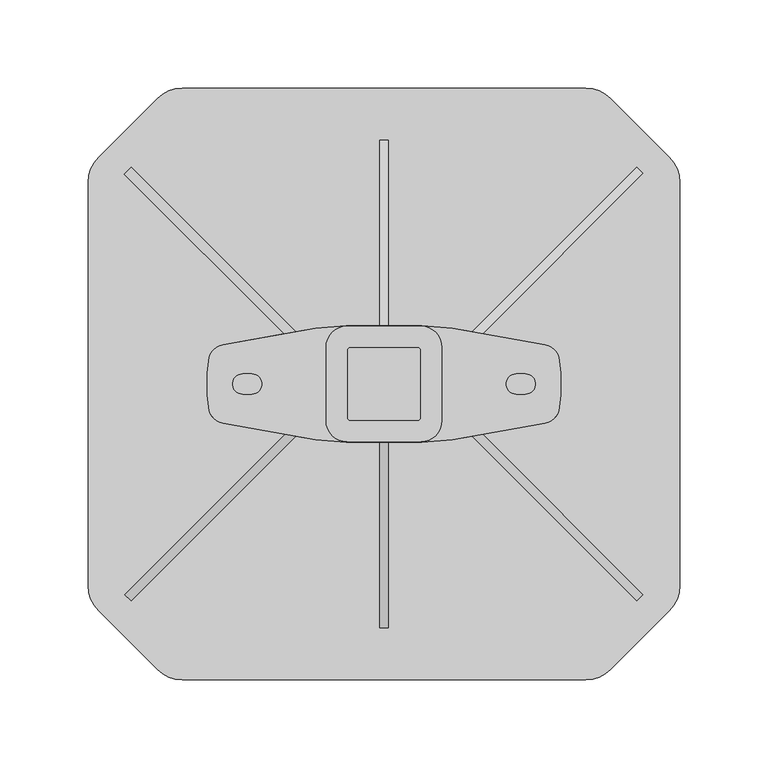
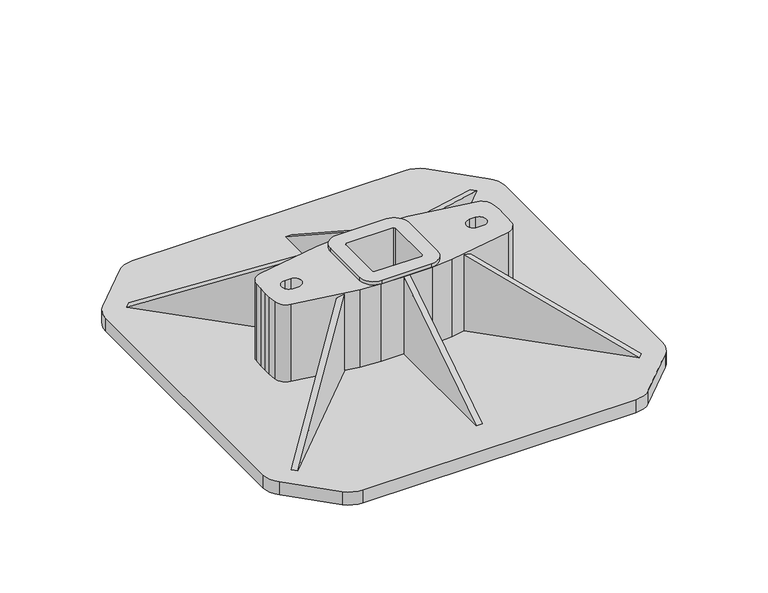
"""IFC4 building model written with IfcOpenShell, lengths in millimetres: proxy geometry, TN_Опора 335 B41-42 : Опора 335 B41/42."""

import ifcopenshell
import ifcopenshell.guid

model = None  # the IFC model being written
_history = None  # IfcOwnerHistory: only IFC2X3 demands one
_inside = {}  # id of a spatial element -> (the spatial element, [elements in it])
_under = {}  # id of a project, library or spatial element -> (it, [spatial elements below it])
_declared = {}  # id of a project -> (the project, [libraries it declares])
_typed = {}  # id of a type object -> (the type object, [elements of that type])
_made_of = {}  # id of a material, layer set ... -> (it, [elements and type objects made of it])


def new_model(schema):
    """Start an empty IFC model of exactly this schema.

    Asked for "IFC4X3", IfcOpenShell would pick the latest addendum, in which some entities
    have other attributes; the version numbers below select the first issue.
    IFC2X3 requires an IfcOwnerHistory on every rooted entity: one is made here for all.
    """
    global model, _history
    if schema == "IFC4X3":
        model = ifcopenshell.file(schema_version=(4, 3, 0, 0))
    else:
        model = ifcopenshell.file(schema=schema)
    _inside.clear()
    _under.clear()
    _declared.clear()
    _typed.clear()
    _made_of.clear()
    _history = None
    if model.schema == "IFC2X3":
        org = make("IfcOrganization", Name="unknown")
        user = make(
            "IfcPersonAndOrganization",
            ThePerson=make("IfcPerson", FamilyName="unknown"),
            TheOrganization=org,
        )
        app = make(
            "IfcApplication",
            ApplicationDeveloper=org,
            Version="unknown",
            ApplicationFullName="unknown",
            ApplicationIdentifier="unknown",
        )
        _history = make(
            "IfcOwnerHistory",
            OwningUser=user,
            OwningApplication=app,
            ChangeAction="ADDED",
            CreationDate=0,
        )
    return model


def make(cls, **values):
    """One entity of the class cls with the attributes given. An attribute that is None is left unset."""
    return model.create_entity(
        cls, **{name: value for name, value in values.items() if value is not None}
    )


def rooted(cls, **values):
    """An entity with a GlobalId (a new one), such as an element, a storey or a relation."""
    return make(cls, GlobalId=ifcopenshell.guid.new(), OwnerHistory=_history, **values)


def si_unit(unit_type, name, prefix=None):
    """IfcSIUnit, for example si_unit("LENGTHUNIT", "METRE", prefix="MILLI")."""
    return make("IfcSIUnit", UnitType=unit_type, Prefix=prefix, Name=name)


def assignment(units):
    """IfcUnitAssignment: the units of a project."""
    return None if units is None else make("IfcUnitAssignment", Units=units)


def point(xyz):
    """IfcCartesianPoint."""
    return None if xyz is None else make("IfcCartesianPoint", Coordinates=xyz)


def direction(xyz):
    """IfcDirection."""
    return None if xyz is None else make("IfcDirection", DirectionRatios=xyz)


def frame(location, z_axis=None, x_axis=None):
    """IfcAxis2Placement3D, a coordinate frame: its origin and axes. An axis left out is left unset."""
    return make(
        "IfcAxis2Placement3D",
        Location=point(location),
        Axis=direction(z_axis),
        RefDirection=direction(x_axis),
    )


def origin():
    """The frame at (0, 0, 0) with its axes left unset."""
    return frame((0.0, 0.0, 0.0))


def place(relative_to, where):
    """IfcLocalPlacement: puts the frame where relative to a parent placement (None: the world)."""
    return make(
        "IfcLocalPlacement", PlacementRelTo=relative_to, RelativePlacement=where
    )


def context(
    kind, dimensions, precision=None, world=None, true_north=None, identifier=None
):
    """IfcGeometricRepresentationContext, for example the 3D "Model" context."""
    return make(
        "IfcGeometricRepresentationContext",
        ContextIdentifier=identifier,
        ContextType=kind,
        CoordinateSpaceDimension=dimensions,
        Precision=precision,
        WorldCoordinateSystem=world,
        TrueNorth=true_north,
    )


def project(units=None, contexts=None):
    """IfcProject with its units and contexts."""
    return rooted(
        "IfcProject",
        Name="project",
        RepresentationContexts=contexts,
        UnitsInContext=assignment(units),
    )


def spatial(cls, under=None, at=None, **own):
    """A site, building, storey or space (cls), placed at a placement, below another one or the project."""
    s = rooted(cls, ObjectPlacement=at, **own)
    if under is not None:
        _under.setdefault(under.id(), (under, []))[1].append(s)
    return s


def polyline(points):
    """IfcPolyline through the points."""
    return make("IfcPolyline", Points=[point(p) for p in points])


def circle_curve(where, radius):
    """IfcCircle in the frame where."""
    return make("IfcCircle", Position=where, Radius=radius)


def shape(context_of_items, identifier, shape_type, items):
    """IfcShapeRepresentation: the items that make up one representation, for example the "Body"."""
    return make(
        "IfcShapeRepresentation",
        ContextOfItems=context_of_items,
        RepresentationIdentifier=identifier,
        RepresentationType=shape_type,
        Items=items,
    )


def source(mapping_origin, context_of_items, identifier, shape_type, items):
    """IfcRepresentationMap: a shape defined once, which mapped items show again and again."""
    return make(
        "IfcRepresentationMap",
        MappingOrigin=mapping_origin,
        MappedRepresentation=shape(context_of_items, identifier, shape_type, items),
    )


def transform(
    local_origin,
    x_axis=None,
    y_axis=None,
    z_axis=None,
    scale=None,
    scale2=None,
    scale3=None,
    uniform=True,
):
    """IfcCartesianTransformationOperator3D, or its non-uniform kind. x_axis, y_axis, z_axis: its Axis1, 2, 3."""
    if uniform:
        return make(
            "IfcCartesianTransformationOperator3D",
            Axis1=direction(x_axis),
            Axis2=direction(y_axis),
            LocalOrigin=point(local_origin),
            Scale=scale,
            Axis3=direction(z_axis),
        )
    return make(
        "IfcCartesianTransformationOperator3DnonUniform",
        Axis1=direction(x_axis),
        Axis2=direction(y_axis),
        LocalOrigin=point(local_origin),
        Scale=scale,
        Axis3=direction(z_axis),
        Scale2=scale2,
        Scale3=scale3,
    )


def mapped(mapping_source, mapping_target):
    """IfcMappedItem: shows the shape of a source again, moved by a transform."""
    return make(
        "IfcMappedItem", MappingSource=mapping_source, MappingTarget=mapping_target
    )


def made_of(thing, what):
    """Note that an element or type object is made of a material, layer set ...; save() writes the relation."""
    if what is not None:
        _made_of.setdefault(what.id(), (what, []))[1].append(thing)
    return thing


def element(
    cls,
    number,
    at=None,
    inside=None,
    cuts=None,
    type_object=None,
    material=None,
    context=None,
    identifier="Body",
    shape_type=None,
    held_by="IfcProductDefinitionShape",
    body=None,
    shapes=None,
    **own,
):
    """One element of the class cls, such as IfcWall. Its Tag is "e" and its number.

    at: its placement. inside: the storey or other place that contains it. cuts: it is an
    opening in that element (IfcRelVoidsElement). A single representation is given by context,
    identifier, shape_type and body (its items); several are given by shapes. held_by: the class
    of the entity that holds the representations. save() writes the other relations.
    """
    e = rooted(cls, Tag="e%d" % number, ObjectPlacement=at, **own)
    if body is not None:
        shapes = [shape(context, identifier, shape_type, body)]
    if shapes is not None:
        e.Representation = make(held_by, Representations=shapes)
    if inside is not None:
        _inside.setdefault(inside.id(), (inside, []))[1].append(e)
    if cuts is not None:
        rooted(
            "IfcRelVoidsElement", RelatingBuildingElement=cuts, RelatedOpeningElement=e
        )
    if type_object is not None:
        _typed.setdefault(type_object.id(), (type_object, []))[1].append(e)
    return made_of(e, material)


def aggregate(whole, parts):
    """IfcRelAggregates: a whole, such as a stair, and the parts it consists of."""
    return rooted("IfcRelAggregates", RelatingObject=whole, RelatedObjects=parts)


def save(model, path):
    """Write the relations noted so far, then the file.

    IfcRelAggregates (storeys below a building ...), IfcRelContainedInSpatialStructure (elements
    in a storey), IfcRelDefinesByType, IfcRelAssociatesMaterial and IfcRelDeclares: one each for
    every whole, place, type object, material and project.
    """
    for whole, parts in _under.values():
        aggregate(whole, parts)
    for where, things in _inside.values():
        rooted(
            "IfcRelContainedInSpatialStructure",
            RelatedElements=things,
            RelatingStructure=where,
        )
    for kind, things in _typed.values():
        rooted("IfcRelDefinesByType", RelatedObjects=things, RelatingType=kind)
    for what, things in _made_of.values():
        rooted("IfcRelAssociatesMaterial", RelatedObjects=things, RelatingMaterial=what)
    for by, libraries in _declared.values():
        rooted("IfcRelDeclares", RelatingContext=by, RelatedDefinitions=libraries)
    model.write(path)


def plane_surface(at):
    """IfcPlane: the flat surface through the origin of the frame at, square to its z axis."""
    return make("IfcPlane", Position=at)


def cylinder_surface(at, radius):
    """IfcCylindricalSurface: all points at the distance radius from the z axis of the frame at."""
    return make("IfcCylindricalSurface", Position=at, Radius=radius)


def revolved_surface(curve, axis_point, axis_direction):
    """IfcSurfaceOfRevolution: the curve turned about the line through axis_point along axis_direction."""
    return make(
        "IfcSurfaceOfRevolution",
        SweptCurve=make("IfcArbitraryOpenProfileDef", ProfileType="CURVE", Curve=curve),
        AxisPosition=make("IfcAxis1Placement", Location=point(axis_point), Axis=direction(axis_direction)),
    )


def advanced_brep(points, edges, surfaces, faces):
    """IfcAdvancedBrep: a solid bounded by faces that lie on surfaces and meet in shared edges.

    An edge is (start, end): straight between two places in points (the first is 0);
    or (start, end, curve); or (start, end, curve, False) where it runs against its curve.
    A face is (place in surfaces, loops), or (place, loops, False) where it looks against
    its surface's normal. A loop lists edges by number (the first is 1), with a minus sign
    where the edge is run from its end to its start. The first loop is the outer one.
    """
    corners = [point(p) for p in points]
    vertices = [make("IfcVertexPoint", VertexGeometry=c) for c in corners]
    made = []
    for start, end, *more in edges:
        made.append(
            make(
                "IfcEdgeCurve",
                EdgeStart=vertices[start],
                EdgeEnd=vertices[end],
                EdgeGeometry=more[0] if more else make("IfcPolyline", Points=[corners[start], corners[end]]),
                SameSense=more[1] if len(more) > 1 else True,
            )
        )
    hull = []
    for where, loops, *sense in faces:
        bounds = []
        for j, loop in enumerate(loops):
            ring = [make("IfcOrientedEdge", EdgeElement=made[abs(k) - 1], Orientation=k > 0) for k in loop]
            bounds.append(
                make(
                    "IfcFaceOuterBound" if j == 0 else "IfcFaceBound",
                    Bound=make("IfcEdgeLoop", EdgeList=ring),
                    Orientation=True,
                )
            )
        hull.append(make("IfcAdvancedFace", Bounds=bounds, FaceSurface=surfaces[where], SameSense=sense[0] if sense else True))
    return make("IfcAdvancedBrep", Outer=make("IfcClosedShell", CfsFaces=hull))


def generic_models_af6bc42f(model_context):
    return source(origin(), model_context, "Body", "AdvancedBrep", [
        advanced_brep(
        [(-23.35, -19.35, 11.5), (-23.35, 19.35, 11.5), (-19.35, 23.35, 11.5), (19.35, 23.35, 11.5), (23.35, 19.35, 11.5), (23.35, -19.35, 11.5), (19.35, -23.35, 11.5), (-19.35, -23.35, 11.5), (-19.5893398, 20.65, 11.5), (-20.65, 19.5893398, 11.5), (-20.65, -19.5893398, 11.5), (-19.5893398, -20.65, 11.5), (19.5893398, -20.65, 11.5), (20.65, -19.5893398, 11.5), (20.65, 19.5893398, 11.5), (19.5893398, 20.65, 11.5), (-19.35, -23.35, 80.0), (-23.35, -19.35, 80.0), (19.35, -23.35, 80.0), (23.35, -19.35, 80.0), (23.35, 19.35, 80.0), (19.35, 23.35, 80.0), (-19.35, 23.35, 80.0), (-23.35, 19.35, 80.0), (19.5893398, 20.65, 83.0), (-19.5893398, 20.65, 83.0), (20.65, 19.5893398, 83.0), (20.65, -19.5893398, 83.0), (19.5893398, -20.65, 83.0), (-19.5893398, -20.65, 83.0), (-20.65, -19.5893398, 83.0), (-20.65, 19.5893398, 83.0), (-32.8, 20.8, 83.0), (-32.8, -20.8, 83.0), (-20.8, -32.8, 83.0), (20.8, -32.8, 83.0), (32.8, -20.8, 83.0), (32.8, 20.8, 83.0), (20.8, 32.8, 83.0), (-20.8, 32.8, 83.0), (-32.8, 20.8, 80.0), (-20.8, 32.8, 80.0), (20.8, 32.8, 80.0), (32.8, 20.8, 80.0), (32.8, -20.8, 80.0), (20.8, -32.8, 80.0), (-20.8, -32.8, 80.0), (-32.8, -20.8, 80.0)],
        [
            (0, 1),
            (1, 2, circle_curve(frame((-19.35, 19.35, 11.5), z_axis=(0.0, 0.0, -1.0), x_axis=(1.0, 0.0, 0.0)), 4.0)),
            (2, 3),
            (3, 4, circle_curve(frame((19.35, 19.35, 11.5), z_axis=(0.0, 0.0, -1.0), x_axis=(1.0, 0.0, 0.0)), 4.0)),
            (4, 5),
            (5, 6, circle_curve(frame((19.35, -19.35, 11.5), z_axis=(0.0, 0.0, -1.0), x_axis=(1.0, 0.0, 0.0)), 4.0)),
            (6, 7),
            (7, 0, circle_curve(frame((-19.35, -19.35, 11.5), z_axis=(0.0, 0.0, -1.0), x_axis=(1.0, 0.0, 0.0)), 4.0)),
            (8, 9),
            (9, 10),
            (10, 11),
            (11, 12),
            (12, 13),
            (13, 14),
            (14, 15),
            (15, 8),
            (7, 16),
            (16, 17, circle_curve(frame((-19.35, -19.35, 80.0), z_axis=(0.0, 0.0, -1.0), x_axis=(1.0, 0.0, 0.0)), 4.0)),
            (17, 0),
            (6, 18),
            (18, 16),
            (5, 19),
            (19, 18, circle_curve(frame((19.35, -19.35, 80.0), z_axis=(0.0, 0.0, -1.0), x_axis=(1.0, 0.0, 0.0)), 4.0)),
            (4, 20),
            (20, 19),
            (3, 21),
            (21, 20, circle_curve(frame((19.35, 19.35, 80.0), z_axis=(0.0, 0.0, -1.0), x_axis=(1.0, 0.0, 0.0)), 4.0)),
            (2, 22),
            (22, 21),
            (1, 23),
            (23, 22, circle_curve(frame((-19.35, 19.35, 80.0), z_axis=(0.0, 0.0, -1.0), x_axis=(1.0, 0.0, 0.0)), 4.0)),
            (17, 23),
            (15, 24),
            (24, 25),
            (25, 8),
            (14, 26),
            (26, 24),
            (13, 27),
            (27, 26),
            (12, 28),
            (28, 27),
            (11, 29),
            (29, 28),
            (10, 30),
            (30, 29),
            (9, 31),
            (31, 30),
            (25, 31),
            (32, 33),
            (33, 34, circle_curve(frame((-20.8, -20.8, 83.0), z_axis=(0.0, 0.0, 1.0), x_axis=(1.0, 0.0, 0.0)), 12.0)),
            (34, 35),
            (35, 36, circle_curve(frame((20.8, -20.8, 83.0), z_axis=(0.0, 0.0, 1.0), x_axis=(1.0, 0.0, 0.0)), 12.0)),
            (36, 37),
            (37, 38, circle_curve(frame((20.8, 20.8, 83.0), z_axis=(0.0, 0.0, 1.0), x_axis=(1.0, 0.0, 0.0)), 12.0)),
            (38, 39),
            (39, 32, circle_curve(frame((-20.8, 20.8, 83.0), z_axis=(0.0, 0.0, 1.0), x_axis=(1.0, 0.0, 0.0)), 12.0)),
            (40, 41, circle_curve(frame((-20.8, 20.8, 80.0), z_axis=(0.0, 0.0, -1.0), x_axis=(1.0, 0.0, 0.0)), 12.0)),
            (41, 42),
            (42, 43, circle_curve(frame((20.8, 20.8, 80.0), z_axis=(0.0, 0.0, -1.0), x_axis=(1.0, 0.0, 0.0)), 12.0)),
            (43, 44),
            (44, 45, circle_curve(frame((20.8, -20.8, 80.0), z_axis=(0.0, 0.0, -1.0), x_axis=(1.0, 0.0, 0.0)), 12.0)),
            (45, 46),
            (46, 47, circle_curve(frame((-20.8, -20.8, 80.0), z_axis=(0.0, 0.0, -1.0), x_axis=(1.0, 0.0, 0.0)), 12.0)),
            (47, 40),
            (32, 40),
            (47, 33),
            (46, 34),
            (45, 35),
            (44, 36),
            (43, 37),
            (42, 38),
            (41, 39),
        ],
        [
            plane_surface(frame((-15.35, -19.35, 11.5), z_axis=(0.0, 0.0, -1.0), x_axis=(0.0, -1.0, 0.0))),
            cylinder_surface(frame((-19.35, -19.35, 11.5), z_axis=(0.0, 0.0, 1.0), x_axis=(1.0, 0.0, 0.0)), 4.0),
            plane_surface(frame((-19.35, -23.35, 80.0), z_axis=(0.0, -1.0, 0.0), x_axis=(0.0, 0.0, -1.0))),
            cylinder_surface(frame((19.35, -19.35, 11.5), z_axis=(0.0, 0.0, 1.0), x_axis=(1.0, 0.0, 0.0)), 4.0),
            plane_surface(frame((23.35, -19.35, 80.0), z_axis=(1.0, 0.0, 0.0), x_axis=(0.0, 0.0, -1.0))),
            cylinder_surface(frame((19.35, 19.35, 11.5), z_axis=(0.0, 0.0, 1.0), x_axis=(1.0, 0.0, 0.0)), 4.0),
            plane_surface(frame((19.35, 23.35, 80.0), z_axis=(0.0, 1.0, 0.0), x_axis=(0.0, 0.0, -1.0))),
            cylinder_surface(frame((-19.35, 19.35, 11.5), z_axis=(0.0, 0.0, 1.0), x_axis=(1.0, 0.0, 0.0)), 4.0),
            plane_surface(frame((-23.35, 19.35, 80.0), z_axis=(-1.0, 0.0, 0.0), x_axis=(0.0, 0.0, -1.0))),
            plane_surface(frame((-19.5893398, 20.65, 80.0), z_axis=(0.0, -1.0, 0.0), x_axis=(0.0, 0.0, -1.0))),
            plane_surface(frame((19.5893398, 20.65, 80.0), z_axis=(-0.7071067811865461, -0.707106781186549, 0.0), x_axis=(0.0, 0.0, -1.0))),
            plane_surface(frame((20.65, 19.5893398, 80.0), z_axis=(-1.0, 0.0, 0.0), x_axis=(0.0, 0.0, -1.0))),
            plane_surface(frame((20.65, -19.5893398, 80.0), z_axis=(-0.7071067811865461, 0.7071067811865489, 0.0), x_axis=(0.0, 0.0, -1.0))),
            plane_surface(frame((19.5893398, -20.65, 80.0), z_axis=(0.0, 1.0, 0.0), x_axis=(0.0, 0.0, -1.0))),
            plane_surface(frame((-19.5893398, -20.65, 80.0), z_axis=(0.707106781186549, 0.7071067811865461, 0.0), x_axis=(0.0, 0.0, -1.0))),
            plane_surface(frame((-20.65, -19.5893398, 80.0), z_axis=(1.0, 0.0, 0.0), x_axis=(0.0, 0.0, -1.0))),
            plane_surface(frame((-20.65, 19.5893398, 80.0), z_axis=(0.7071067811865476, -0.7071067811865476, 0.0), x_axis=(0.0, 0.0, -1.0))),
            plane_surface(frame((-20.65, 19.5893398, 83.0), z_axis=(0.0, 0.0, 1.0000000000000002), x_axis=(0.7071067811865462, 0.707106781186549, 0.0))),
            plane_surface(frame((-20.65, 19.5893398, 80.0), z_axis=(0.0, 0.0, -1.0000000000000002), x_axis=(-0.7071067811865462, -0.707106781186549, 0.0))),
            plane_surface(frame((-32.8, 20.8, 83.0), z_axis=(-1.0, 0.0, 0.0), x_axis=(0.0, 0.0, -1.0))),
            cylinder_surface(frame((-20.8, -20.8, 15.5), z_axis=(0.0, 0.0, 1.0), x_axis=(1.0, 0.0, 0.0)), 12.0),
            plane_surface(frame((-20.8, -32.8, 83.0), z_axis=(0.0, -1.0, 0.0), x_axis=(0.0, 0.0, -1.0))),
            cylinder_surface(frame((20.8, -20.8, 15.5), z_axis=(0.0, 0.0, 1.0), x_axis=(1.0, 0.0, 0.0)), 12.0),
            plane_surface(frame((32.8, -20.8, 83.0), z_axis=(1.0, 0.0, 0.0), x_axis=(0.0, 0.0, -1.0))),
            cylinder_surface(frame((20.8, 20.8, 15.5), z_axis=(0.0, 0.0, 1.0), x_axis=(1.0, 0.0, 0.0)), 12.0),
            plane_surface(frame((20.8, 32.8, 83.0), z_axis=(0.0, 1.0, 0.0), x_axis=(0.0, 0.0, -1.0))),
            cylinder_surface(frame((-20.8, 20.8, 15.5), z_axis=(0.0, 0.0, 1.0), x_axis=(1.0, 0.0, 0.0)), 12.0),
        ],
        [
            (0, [[1, 2, 3, 4, 5, 6, 7, 8], [9, 10, 11, 12, 13, 14, 15, 16]]),
            (1, [[-8, 17, 18, 19]]),
            (2, [[-7, 20, 21, -17]]),
            (3, [[-6, 22, 23, -20]]),
            (4, [[-5, 24, 25, -22]]),
            (5, [[-4, 26, 27, -24]]),
            (6, [[-3, 28, 29, -26]]),
            (7, [[-2, 30, 31, -28]]),
            (8, [[-1, -19, 32, -30]]),
            (9, [[-16, 33, 34, 35]]),
            (10, [[-33, -15, 36, 37]]),
            (11, [[-36, -14, 38, 39]]),
            (12, [[-38, -13, 40, 41]]),
            (13, [[-40, -12, 42, 43]]),
            (14, [[-42, -11, 44, 45]]),
            (15, [[-44, -10, 46, 47]]),
            (16, [[-46, -9, -35, 48]]),
            (17, [[49, 50, 51, 52, 53, 54, 55, 56], [-48, -34, -37, -39, -41, -43, -45, -47]]),
            (18, [[57, 58, 59, 60, 61, 62, 63, 64], [-18, -21, -23, -25, -27, -29, -31, -32]]),
            (19, [[-49, 65, -64, 66]]),
            (20, [[-50, -66, -63, 67]]),
            (21, [[-51, -67, -62, 68]]),
            (22, [[-52, -68, -61, 69]]),
            (23, [[-53, -69, -60, 70]]),
            (24, [[-54, -70, -59, 71]]),
            (25, [[-55, -71, -58, 72]]),
            (26, [[-56, -72, -57, -65]]),
        ],
    ),
        advanced_brep(
        [(-143.1614178, 122.7969517, 11.5), (-49.8622207, 29.4977546, 79.0270484), (-49.8622207, 29.4977546, 11.5), (-56.4807324, 28.3307324, 77.0542393), (-147.0541847, 118.9041847, 11.5), (-56.4807324, 28.3307324, 11.5), (21.2511336, -33.0, 80.0), (38.6159514, -31.4807753, 80.0), (91.1408813, -22.219213, 80.0), (99.3663465, -13.2426929, 80.0), (100.0, -6.0, 80.0), (100.0, 0.0, 80.0), (100.0, 6.0, 80.0), (99.3663465, 13.2426929, 80.0), (91.1408813, 22.219213, 80.0), (38.6159514, 31.4807753, 80.0), (21.2511336, 33.0, 80.0), (2.5, 33.0, 80.0), (0.0, 33.0, 80.0), (-2.5, 33.0, 80.0), (-21.2511336, 33.0, 80.0), (-38.6159514, 31.4807753, 80.0), (-91.1408813, 22.219213, 80.0), (-99.3663465, 13.2426929, 80.0), (-100.0, 6.0, 80.0), (-100.0, 0.0, 80.0), (-100.0, -6.0, 80.0), (-99.3663465, -13.2426929, 80.0), (-91.1408813, -22.219213, 80.0), (-38.6159514, -31.4807753, 80.0), (-21.2511336, -33.0, 80.0), (-2.5, -33.0, 80.0), (0.0, -33.0, 80.0), (2.5, -33.0, 80.0), (-80.0, -5.75, 80.0), (-80.0, 5.75, 80.0), (-75.0, 5.75, 80.0), (-75.0, -5.75, 80.0), (80.0, -5.75, 80.0), (75.0, -5.75, 80.0), (75.0, 5.75, 80.0), (80.0, 5.75, 80.0), (-4.25, 25.0, 80.0), (-4.25, 23.9, 80.0), (4.25, 23.9, 80.0), (4.25, 25.0, 80.0), (25.0, 25.0, 80.0), (25.0, 4.25, 80.0), (23.9, 4.25, 80.0), (23.9, -4.25, 80.0), (25.0, -4.25, 80.0), (25.0, -25.0, 80.0), (4.25, -25.0, 80.0), (4.25, -23.9, 80.0), (-4.25, -23.9, 80.0), (-4.25, -25.0, 80.0), (-25.0, -25.0, 80.0), (-25.0, -4.25, 80.0), (-23.9, -4.25, 80.0), (-23.9, 4.25, 80.0), (-25.0, 4.25, 80.0), (-25.0, 25.0, 80.0), (-80.0, -5.75, 11.5), (-80.0, 5.75, 11.5), (-75.0, 5.75, 11.5), (-75.0, -5.75, 11.5), (80.0, -5.75, 11.5), (75.0, -5.75, 11.5), (75.0, 5.75, 11.5), (80.0, 5.75, 11.5), (-21.2511336, -33.0, 11.5), (-2.5, -33.0, 11.5), (21.2511336, -33.0, 11.5), (2.5, -33.0, 11.5), (38.6159514, -31.4807753, 11.5), (49.8622207, -29.4977546, 11.5), (49.8622207, -29.4977546, 79.0270484), (55.8733621, -28.4378282, 77.2352809), (55.8733621, -28.4378282, 11.5), (91.1408813, -22.219213, 11.5), (99.3663465, -13.2426929, 11.5), (100.0, -6.0, 11.5), (100.0, 0.0, 11.5), (100.0, 6.0, 11.5), (99.3663465, 13.2426929, 11.5), (91.1408813, 22.219213, 11.5), (55.8733621, 28.4378282, 11.5), (55.8733621, 28.4378282, 77.2352809), (49.8622207, 29.4977546, 79.0270484), (49.8622207, 29.4977546, 11.5), (38.6159514, 31.4807753, 11.5), (21.2511336, 33.0, 11.5), (2.5, 33.0, 11.5), (-21.2511336, 33.0, 11.5), (-2.5, 33.0, 11.5), (-38.6159514, 31.4807753, 11.5), (-91.1408813, 22.219213, 11.5), (-99.3663465, 13.2426929, 11.5), (-100.0, 6.0, 11.5), (-100.0, 0.0, 11.5), (-100.0, -6.0, 11.5), (-99.3663465, -13.2426929, 11.5), (-91.1408813, -22.219213, 11.5), (-55.8733621, -28.4378282, 11.5), (-55.8733621, -28.4378282, 77.2352809), (-49.8622207, -29.4977546, 79.0270484), (-49.8622207, -29.4977546, 11.5), (-38.6159514, -31.4807753, 11.5), (-4.25, 25.0, 11.5), (-4.25, 23.9, 11.5), (4.25, 23.9, 11.5), (4.25, 25.0, 11.5), (25.0, 25.0, 11.5), (25.0, 4.25, 11.5), (23.9, 4.25, 11.5), (23.9, -4.25, 11.5), (25.0, -4.25, 11.5), (25.0, -25.0, 11.5), (4.25, -25.0, 11.5), (4.25, -23.9, 11.5), (-4.25, -23.9, 11.5), (-4.25, -25.0, 11.5), (-25.0, -25.0, 11.5), (-25.0, -4.25, 11.5), (-23.9, -4.25, 11.5), (-23.9, 4.25, 11.5), (-25.0, 4.25, 11.5), (-25.0, 25.0, 11.5), (2.5, 138.0, 11.5), (-2.5, 138.0, 11.5), (143.1614178, 122.7969517, 11.5), (146.6969517, 119.2614178, 11.5), (143.1614178, -122.7969517, 11.5), (146.6969517, -119.2614178, 11.5), (2.5, -138.0, 11.5), (-2.5, -138.0, 11.5), (-143.1614178, -122.7969517, 11.5), (-146.6969517, -119.2614178, 11.5), (114.2157288, 167.5, 11.5), (-114.2157288, 167.5, 11.5), (-128.3578644, 161.6421356, 11.5), (-161.6421356, 128.3578644, 11.5), (-167.5, 114.2157288, 11.5), (-167.5, -114.2157288, 11.5), (-161.6421356, -128.3578644, 11.5), (-128.3578644, -161.6421356, 11.5), (-114.2157288, -167.5, 11.5), (114.2157288, -167.5, 11.5), (128.3578644, -161.6421356, 11.5), (161.6421356, -128.3578644, 11.5), (167.5, -114.2157288, 11.5), (167.5, 114.2157288, 11.5), (161.6421356, 128.3578644, 11.5), (128.3578644, 161.6421356, 11.5), (114.2157288, 167.5, 0.0), (128.3578644, 161.6421356, 0.0), (161.6421356, 128.3578644, 0.0), (167.5, 114.2157288, 0.0), (167.5, -114.2157288, 0.0), (161.6421356, -128.3578644, 0.0), (128.3578644, -161.6421356, 0.0), (114.2157288, -167.5, 0.0), (-114.2157288, -167.5, 0.0), (-128.3578644, -161.6421356, 0.0), (-161.6421356, -128.3578644, 0.0), (-167.5, -114.2157288, 0.0), (-167.5, 114.2157288, 0.0), (-161.6421356, 128.3578644, 0.0), (-128.3578644, 161.6421356, 0.0), (-114.2157288, 167.5, 0.0)],
        [
            (0, 1),
            (1, 2),
            (2, 0),
            (3, 4),
            (4, 5),
            (5, 3),
            (0, 4),
            (3, 1),
            (6, 7, circle_curve(frame((21.2511336, 67.0, 80.0), z_axis=(0.0, 0.0, 1.0), x_axis=(1.0, 0.0, 0.0)), 100.0)),
            (7, 8),
            (8, 9, circle_curve(frame((89.4043995, -12.3711355, 80.0), z_axis=(0.0, 0.0, 1.0), x_axis=(1.0, 0.0, 0.0)), 10.0)),
            (9, 10),
            (10, 11),
            (11, 12),
            (12, 13),
            (13, 14, circle_curve(frame((89.4043995, 12.3711355, 80.0), z_axis=(0.0, 0.0, 1.0), x_axis=(1.0, 0.0, 0.0)), 10.0)),
            (14, 15),
            (15, 16, circle_curve(frame((21.2511336, -67.0, 80.0), z_axis=(0.0, 0.0, 1.0), x_axis=(1.0, 0.0, 0.0)), 100.0)),
            (16, 17),
            (17, 18),
            (18, 19),
            (19, 20),
            (20, 21, circle_curve(frame((-21.2511336, -67.0, 80.0), z_axis=(0.0, 0.0, 1.0), x_axis=(1.0, 0.0, 0.0)), 100.0)),
            (21, 22),
            (22, 23, circle_curve(frame((-89.4043995, 12.3711355, 80.0), z_axis=(0.0, 0.0, 1.0), x_axis=(1.0, 0.0, 0.0)), 10.0)),
            (23, 24),
            (24, 25),
            (25, 26),
            (26, 27),
            (27, 28, circle_curve(frame((-89.4043995, -12.3711355, 80.0), z_axis=(0.0, 0.0, 1.0), x_axis=(1.0, 0.0, 0.0)), 10.0)),
            (28, 29),
            (29, 30, circle_curve(frame((-21.2511336, 67.0, 80.0), z_axis=(0.0, 0.0, 1.0), x_axis=(1.0, 0.0, 0.0)), 100.0)),
            (30, 31),
            (31, 32),
            (32, 33),
            (33, 6),
            (34, 35, circle_curve(frame((-80.0, 0.0, 80.0), z_axis=(0.0, 0.0, -1.0), x_axis=(1.0, 0.0, 0.0)), 5.75)),
            (35, 36),
            (36, 37, circle_curve(frame((-75.0, 0.0, 80.0), z_axis=(0.0, 0.0, -1.0), x_axis=(1.0, 0.0, 0.0)), 5.75)),
            (37, 34),
            (38, 39),
            (39, 40, circle_curve(frame((75.0, 0.0, 80.0), z_axis=(0.0, 0.0, -1.0), x_axis=(1.0, 0.0, 0.0)), 5.75)),
            (40, 41),
            (41, 38, circle_curve(frame((80.0, 0.0, 80.0), z_axis=(0.0, 0.0, -1.0), x_axis=(1.0, 0.0, 0.0)), 5.75)),
            (42, 43),
            (43, 44),
            (44, 45),
            (45, 46),
            (46, 47),
            (47, 48),
            (48, 49),
            (49, 50),
            (50, 51),
            (51, 52),
            (52, 53),
            (53, 54),
            (54, 55),
            (55, 56),
            (56, 57),
            (57, 58),
            (58, 59),
            (59, 60),
            (60, 61),
            (61, 42),
            (34, 62),
            (62, 63, circle_curve(frame((-80.0, 0.0, 11.5), z_axis=(0.0, 0.0, -1.0), x_axis=(1.0, 0.0, 0.0)), 5.75)),
            (63, 35),
            (63, 64),
            (64, 36),
            (64, 65, circle_curve(frame((-75.0, 0.0, 11.5), z_axis=(0.0, 0.0, -1.0), x_axis=(1.0, 0.0, 0.0)), 5.75)),
            (65, 37),
            (65, 62),
            (38, 66),
            (66, 67),
            (67, 39),
            (67, 68, circle_curve(frame((75.0, 0.0, 11.5), z_axis=(0.0, 0.0, -1.0), x_axis=(1.0, 0.0, 0.0)), 5.75)),
            (68, 40),
            (68, 69),
            (69, 41),
            (69, 66, circle_curve(frame((80.0, 0.0, 11.5), z_axis=(0.0, 0.0, -1.0), x_axis=(1.0, 0.0, 0.0)), 5.75)),
            (30, 70),
            (70, 71),
            (71, 31),
            (72, 6),
            (33, 73),
            (73, 72),
            (72, 74, circle_curve(frame((21.2511336, 67.0, 11.5), z_axis=(0.0, 0.0, 1.0), x_axis=(1.0, 0.0, 0.0)), 100.0)),
            (74, 7),
            (74, 75),
            (75, 76),
            (76, 77),
            (77, 78),
            (78, 79),
            (79, 8),
            (79, 80, circle_curve(frame((89.4043995, -12.3711355, 11.5), z_axis=(0.0, 0.0, 1.0), x_axis=(1.0, 0.0, 0.0)), 10.0)),
            (80, 9),
            (80, 81),
            (81, 10),
            (81, 82),
            (82, 11),
            (82, 83),
            (83, 12),
            (83, 84),
            (84, 13),
            (84, 85, circle_curve(frame((89.4043995, 12.3711355, 11.5), z_axis=(0.0, 0.0, 1.0), x_axis=(1.0, 0.0, 0.0)), 10.0)),
            (85, 14),
            (85, 86),
            (86, 87),
            (87, 88),
            (88, 89),
            (89, 90),
            (90, 15),
            (90, 91, circle_curve(frame((21.2511336, -67.0, 11.5), z_axis=(0.0, 0.0, 1.0), x_axis=(1.0, 0.0, 0.0)), 100.0)),
            (91, 16),
            (91, 92),
            (92, 17),
            (93, 20),
            (19, 94),
            (94, 93),
            (93, 95, circle_curve(frame((-21.2511336, -67.0, 11.5), z_axis=(0.0, 0.0, 1.0), x_axis=(1.0, 0.0, 0.0)), 100.0)),
            (95, 21),
            (95, 2),
            (5, 96),
            (96, 22),
            (96, 97, circle_curve(frame((-89.4043995, 12.3711355, 11.5), z_axis=(0.0, 0.0, 1.0), x_axis=(1.0, 0.0, 0.0)), 10.0)),
            (97, 23),
            (97, 98),
            (98, 24),
            (98, 99),
            (99, 25),
            (99, 100),
            (100, 26),
            (100, 101),
            (101, 27),
            (101, 102, circle_curve(frame((-89.4043995, -12.3711355, 11.5), z_axis=(0.0, 0.0, 1.0), x_axis=(1.0, 0.0, 0.0)), 10.0)),
            (102, 28),
            (102, 103),
            (103, 104),
            (104, 105),
            (105, 106),
            (106, 107),
            (107, 29),
            (107, 70, circle_curve(frame((-21.2511336, 67.0, 11.5), z_axis=(0.0, 0.0, 1.0), x_axis=(1.0, 0.0, 0.0)), 100.0)),
            (42, 108),
            (108, 109),
            (109, 43),
            (109, 110),
            (110, 44),
            (110, 111),
            (111, 45),
            (111, 112),
            (112, 46),
            (112, 113),
            (113, 47),
            (113, 114),
            (114, 48),
            (114, 115),
            (115, 49),
            (115, 116),
            (116, 50),
            (116, 117),
            (117, 51),
            (117, 118),
            (118, 52),
            (118, 119),
            (119, 53),
            (119, 120),
            (120, 54),
            (120, 121),
            (121, 55),
            (121, 122),
            (122, 56),
            (122, 123),
            (123, 57),
            (123, 124),
            (124, 58),
            (124, 125),
            (125, 59),
            (125, 126),
            (126, 60),
            (126, 127),
            (127, 61),
            (127, 108),
            (128, 17),
            (92, 128),
            (19, 129),
            (129, 94),
            (128, 129),
            (88, 130),
            (130, 89),
            (131, 87),
            (86, 131),
            (131, 130),
            (132, 76),
            (75, 132),
            (77, 133),
            (133, 78),
            (132, 133),
            (33, 134),
            (134, 73),
            (135, 31),
            (71, 135),
            (135, 134),
            (105, 136),
            (136, 106),
            (137, 104),
            (103, 137),
            (137, 136),
            (138, 139),
            (139, 140, circle_curve(frame((-114.2157288, 147.5, 11.5), z_axis=(0.0, 0.0, 1.0), x_axis=(1.0, 0.0, 0.0)), 20.0)),
            (140, 141),
            (141, 142, circle_curve(frame((-147.5, 114.2157288, 11.5), z_axis=(0.0, 0.0, 1.0), x_axis=(1.0, 0.0, 0.0)), 20.0)),
            (142, 143),
            (143, 144, circle_curve(frame((-147.5, -114.2157288, 11.5), z_axis=(0.0, 0.0, 1.0), x_axis=(1.0, 0.0, 0.0)), 20.0)),
            (144, 145),
            (145, 146, circle_curve(frame((-114.2157288, -147.5, 11.5), z_axis=(0.0, 0.0, 1.0), x_axis=(1.0, 0.0, 0.0)), 20.0)),
            (146, 147),
            (147, 148, circle_curve(frame((114.2157288, -147.5, 11.5), z_axis=(0.0, 0.0, 1.0), x_axis=(1.0, 0.0, 0.0)), 20.0)),
            (148, 149),
            (149, 150, circle_curve(frame((147.5, -114.2157288, 11.5), z_axis=(0.0, 0.0, 1.0), x_axis=(1.0, 0.0, 0.0)), 20.0)),
            (150, 151),
            (151, 152, circle_curve(frame((147.5, 114.2157288, 11.5), z_axis=(0.0, 0.0, 1.0), x_axis=(1.0, 0.0, 0.0)), 20.0)),
            (152, 153),
            (153, 138, circle_curve(frame((114.2157288, 147.5, 11.5), z_axis=(0.0, 0.0, 1.0), x_axis=(1.0, 0.0, 0.0)), 20.0)),
            (154, 155, circle_curve(frame((114.2157288, 147.5, 0.0), z_axis=(0.0, 0.0, -1.0), x_axis=(1.0, 0.0, 0.0)), 20.0)),
            (155, 156),
            (156, 157, circle_curve(frame((147.5, 114.2157288, 0.0), z_axis=(0.0, 0.0, -1.0), x_axis=(1.0, 0.0, 0.0)), 20.0)),
            (157, 158),
            (158, 159, circle_curve(frame((147.5, -114.2157288, 0.0), z_axis=(0.0, 0.0, -1.0), x_axis=(1.0, 0.0, 0.0)), 20.0)),
            (159, 160),
            (160, 161, circle_curve(frame((114.2157288, -147.5, 0.0), z_axis=(0.0, 0.0, -1.0), x_axis=(1.0, 0.0, 0.0)), 20.0)),
            (161, 162),
            (162, 163, circle_curve(frame((-114.2157288, -147.5, 0.0), z_axis=(0.0, 0.0, -1.0), x_axis=(1.0, 0.0, 0.0)), 20.0)),
            (163, 164),
            (164, 165, circle_curve(frame((-147.5, -114.2157288, 0.0), z_axis=(0.0, 0.0, -1.0), x_axis=(1.0, 0.0, 0.0)), 20.0)),
            (165, 166),
            (166, 167, circle_curve(frame((-147.5, 114.2157288, 0.0), z_axis=(0.0, 0.0, -1.0), x_axis=(1.0, 0.0, 0.0)), 20.0)),
            (167, 168),
            (168, 169, circle_curve(frame((-114.2157288, 147.5, 0.0), z_axis=(0.0, 0.0, -1.0), x_axis=(1.0, 0.0, 0.0)), 20.0)),
            (169, 154),
            (138, 154),
            (169, 139),
            (140, 168),
            (167, 141),
            (142, 166),
            (165, 143),
            (144, 164),
            (163, 145),
            (146, 162),
            (161, 147),
            (148, 160),
            (159, 149),
            (150, 158),
            (157, 151),
            (152, 156),
            (155, 153),
        ],
        [
            plane_surface(frame((-143.1614178, 122.7969517, 11.5), z_axis=(0.7071067811865471, 0.707106781186548, 0.0), x_axis=(0.6294612213167056, -0.6294612213167048, 0.4555843958225127))),
            plane_surface(frame((-147.0541847, 118.9041847, 11.5), z_axis=(-0.7071067811865471, -0.707106781186548, 0.0), x_axis=(-0.6294612213167056, 0.6294612213167048, -0.4555843958225127))),
            plane_surface(frame((-143.1614178, 122.7969517, 11.5), z_axis=(-0.322146815688875, 0.322146815688875, 0.8901925961740168), x_axis=(-0.7071067811865476, -0.7071067811865476, 0.0))),
            plane_surface(frame((-74.25, 0.0, 80.0), z_axis=(0.0, 0.0, 1.0), x_axis=(0.0, -1.0, 0.0))),
            revolved_surface(polyline([(-74.25, 0.0, 11.5), (-74.25, 0.0, 80.0)]), (-80.0, 0.0, 11.5), (0.0, 0.0, -1.0)),
            plane_surface(frame((-80.0, 5.75, 80.0), z_axis=(0.0, -1.0, 0.0), x_axis=(0.0, 0.0, -1.0))),
            revolved_surface(polyline([(-69.25, 0.0, 11.5), (-69.25, 0.0, 80.0)]), (-75.0, 0.0, 11.5), (0.0, 0.0, -1.0)),
            plane_surface(frame((-75.0, -5.75, 80.0), z_axis=(0.0, 1.0, 0.0), x_axis=(0.0, 0.0, -1.0))),
            plane_surface(frame((80.0, -5.75, 80.0), z_axis=(0.0, 1.0, 0.0), x_axis=(0.0, 0.0, -1.0))),
            revolved_surface(polyline([(80.75, 0.0, 11.5), (80.75, 0.0, 80.0)]), (75.0, 0.0, 0.0), (0.0, 0.0, -1.0)),
            plane_surface(frame((75.0, 5.75, 80.0), z_axis=(0.0, -1.0, 0.0), x_axis=(0.0, 0.0, -1.0))),
            revolved_surface(polyline([(85.75, 0.0, 11.5), (85.75, 0.0, 80.0)]), (80.0, 0.0, 0.0), (0.0, 0.0, -1.0)),
            plane_surface(frame((-21.2511336, -33.0, 80.0), z_axis=(0.0, -1.0, 0.0), x_axis=(0.0, 0.0, -1.0))),
            plane_surface(frame((0.0, -33.0, 80.0), z_axis=(0.0, -1.0, 0.0), x_axis=(0.0, 0.0, -1.0))),
            cylinder_surface(frame((21.2511336, 67.0, 0.0), z_axis=(0.0, 0.0, 1.0), x_axis=(1.0, 0.0, 0.0)), 100.0),
            plane_surface(frame((38.6159514, -31.4807753, 80.0), z_axis=(0.17364817766693338, -0.9848077530122076, 0.0), x_axis=(0.0, 0.0, -1.0))),
            cylinder_surface(frame((89.4043995, -12.3711355, 0.0), z_axis=(0.0, 0.0, 1.0), x_axis=(1.0, 0.0, 0.0)), 10.0),
            plane_surface(frame((99.3663465, -13.2426929, 80.0), z_axis=(0.9961946980917454, -0.08715574274765994, 0.0), x_axis=(0.0, 0.0, -1.0))),
            plane_surface(frame((100.0, -6.0, 80.0), z_axis=(1.0, 0.0, 0.0), x_axis=(0.0, 0.0, -1.0))),
            plane_surface(frame((100.0, 0.0, 80.0), z_axis=(1.0, 0.0, 0.0), x_axis=(0.0, 0.0, -1.0))),
            plane_surface(frame((100.0, 6.0, 80.0), z_axis=(0.9961946980917457, 0.08715574274765747, 0.0), x_axis=(0.0, 0.0, -1.0))),
            cylinder_surface(frame((89.4043995, 12.3711355, 0.0), z_axis=(0.0, 0.0, 1.0), x_axis=(1.0, 0.0, 0.0)), 10.0),
            plane_surface(frame((91.1408813, 22.219213, 80.0), z_axis=(0.17364817766693313, 0.9848077530122076, 0.0), x_axis=(0.0, 0.0, -1.0))),
            cylinder_surface(frame((21.2511336, -67.0, 0.0), z_axis=(0.0, 0.0, 1.0), x_axis=(1.0, 0.0, 0.0)), 100.0),
            plane_surface(frame((21.2511336, 33.0, 80.0), z_axis=(0.0, 1.0, 0.0), x_axis=(0.0, 0.0, -1.0))),
            plane_surface(frame((0.0, 33.0, 80.0), z_axis=(0.0, 1.0, 0.0), x_axis=(0.0, 0.0, -1.0))),
            cylinder_surface(frame((-21.2511336, -67.0, 0.0), z_axis=(0.0, 0.0, 1.0), x_axis=(1.0, 0.0, 0.0)), 100.0),
            plane_surface(frame((-38.6159514, 31.4807753, 80.0), z_axis=(-0.17364817766693333, 0.9848077530122076, 0.0), x_axis=(0.0, 0.0, -1.0))),
            cylinder_surface(frame((-89.4043995, 12.3711355, 0.0), z_axis=(0.0, 0.0, 1.0), x_axis=(1.0, 0.0, 0.0)), 10.0),
            plane_surface(frame((-99.3663465, 13.2426929, 80.0), z_axis=(-0.9961946980917454, 0.08715574274765955, 0.0), x_axis=(0.0, 0.0, -1.0))),
            plane_surface(frame((-100.0, 6.0, 80.0), z_axis=(-1.0, 0.0, 0.0), x_axis=(0.0, 0.0, -1.0))),
            plane_surface(frame((-100.0, 0.0, 80.0), z_axis=(-1.0, 0.0, 0.0), x_axis=(0.0, 0.0, -1.0))),
            plane_surface(frame((-100.0, -6.0, 80.0), z_axis=(-0.9961946980917455, -0.08715574274765889, 0.0), x_axis=(0.0, 0.0, -1.0))),
            cylinder_surface(frame((-89.4043995, -12.3711355, 0.0), z_axis=(0.0, 0.0, 1.0), x_axis=(1.0, 0.0, 0.0)), 10.0),
            plane_surface(frame((-91.1408813, -22.219213, 80.0), z_axis=(-0.17364817766693322, -0.9848077530122076, 0.0), x_axis=(0.0, 0.0, -1.0))),
            cylinder_surface(frame((-21.2511336, 67.0, 0.0), z_axis=(0.0, 0.0, 1.0), x_axis=(1.0, 0.0, 0.0)), 100.0),
            plane_surface(frame((-4.25, 25.0, 80.0), z_axis=(-1.0, 0.0, 0.0), x_axis=(0.0, 0.0, -1.0))),
            plane_surface(frame((-4.25, 23.9, 80.0), z_axis=(0.0, -1.0, 0.0), x_axis=(0.0, 0.0, -1.0))),
            plane_surface(frame((4.25, 23.9, 80.0), z_axis=(1.0, 0.0, 0.0), x_axis=(0.0, 0.0, -1.0))),
            plane_surface(frame((4.25, 25.0, 80.0), z_axis=(0.0, -1.0, 0.0), x_axis=(0.0, 0.0, -1.0))),
            plane_surface(frame((25.0, 25.0, 80.0), z_axis=(-1.0, 0.0, 0.0), x_axis=(0.0, 0.0, -1.0))),
            plane_surface(frame((25.0, 4.25, 80.0), z_axis=(0.0, 1.0, 0.0), x_axis=(0.0, 0.0, -1.0))),
            plane_surface(frame((23.9, 4.25, 80.0), z_axis=(-1.0, 0.0, 0.0), x_axis=(0.0, 0.0, -1.0))),
            plane_surface(frame((23.9, -4.25, 80.0), z_axis=(0.0, -1.0, 0.0), x_axis=(0.0, 0.0, -1.0))),
            plane_surface(frame((25.0, -4.25, 80.0), z_axis=(-1.0, 0.0, 0.0), x_axis=(0.0, 0.0, -1.0))),
            plane_surface(frame((25.0, -25.0, 80.0), z_axis=(0.0, 1.0, 0.0), x_axis=(0.0, 0.0, -1.0))),
            plane_surface(frame((4.25, -25.0, 80.0), z_axis=(1.0, 0.0, 0.0), x_axis=(0.0, 0.0, -1.0))),
            plane_surface(frame((4.25, -23.9, 80.0), z_axis=(0.0, 1.0, 0.0), x_axis=(0.0, 0.0, -1.0))),
            plane_surface(frame((-4.25, -23.9, 80.0), z_axis=(-1.0, 0.0, 0.0), x_axis=(0.0, 0.0, -1.0))),
            plane_surface(frame((-4.25, -25.0, 80.0), z_axis=(0.0, 1.0, 0.0), x_axis=(0.0, 0.0, -1.0))),
            plane_surface(frame((-25.0, -25.0, 80.0), z_axis=(1.0, 0.0, 0.0), x_axis=(0.0, 0.0, -1.0))),
            plane_surface(frame((-25.0, -4.25, 80.0), z_axis=(0.0, -1.0, 0.0), x_axis=(0.0, 0.0, -1.0))),
            plane_surface(frame((-23.9, -4.25, 80.0), z_axis=(1.0, 0.0, 0.0), x_axis=(0.0, 0.0, -1.0))),
            plane_surface(frame((-23.9, 4.25, 80.0), z_axis=(0.0, 1.0, 0.0), x_axis=(0.0, 0.0, -1.0))),
            plane_surface(frame((-25.0, 4.25, 80.0), z_axis=(1.0, 0.0, 0.0), x_axis=(0.0, 0.0, -1.0))),
            plane_surface(frame((-25.0, 25.0, 80.0), z_axis=(0.0, -1.0, 0.0), x_axis=(0.0, 0.0, -1.0))),
            plane_surface(frame((2.5, 138.0, 11.5), z_axis=(1.0, 0.0, 0.0), x_axis=(0.0, -0.8375312462789268, 0.5463894320962547))),
            plane_surface(frame((-2.5, 138.0, 11.5), z_axis=(-1.0, 0.0, 0.0), x_axis=(0.0, 0.8375312462789268, -0.5463894320962547))),
            plane_surface(frame((2.5, 138.0, 11.5), z_axis=(0.0, 0.5463894320962547, 0.8375312462789268), x_axis=(-1.0, 0.0, 0.0))),
            plane_surface(frame((65.3796718, 45.0152057, 11.5), z_axis=(-0.7071067811865471, 0.707106781186548, 0.0), x_axis=(-0.707106781186548, -0.7071067811865471, 0.0))),
            plane_surface(frame((68.9152057, 41.4796718, 11.5), z_axis=(0.7071067811865471, -0.707106781186548, 0.0), x_axis=(0.707106781186548, 0.7071067811865471, 0.0))),
            plane_surface(frame((48.5179356, 28.1534695, 80.0), z_axis=(0.3221468156888753, 0.32214681568887454, 0.8901925961740168), x_axis=(0.7071067811865467, -0.7071067811865483, 0.0))),
            plane_surface(frame((48.5179356, -28.1534695, 80.0), z_axis=(-0.707106781186547, -0.7071067811865481, 0.0), x_axis=(-0.6294612213167055, 0.6294612213167045, 0.4555843958225132))),
            plane_surface(frame((52.0534695, -24.6179356, 80.0), z_axis=(0.707106781186547, 0.7071067811865481, 0.0), x_axis=(0.6294612213167055, -0.6294612213167045, -0.4555843958225132))),
            plane_surface(frame((143.1614178, -122.7969517, 11.5), z_axis=(0.3221468156888754, -0.3221468156888754, 0.8901925961740167), x_axis=(0.7071067811865476, 0.7071067811865476, 0.0))),
            plane_surface(frame((2.5, -33.0, 11.5), z_axis=(1.0, 0.0, 0.0), x_axis=(0.0, 1.0, 0.0))),
            plane_surface(frame((-2.5, -33.0, 11.5), z_axis=(-1.0, 0.0, 0.0), x_axis=(0.0, -1.0, 0.0))),
            plane_surface(frame((2.5, -33.0, 80.0), z_axis=(0.0, -0.5463894320962547, 0.8375312462789268), x_axis=(-1.0, 0.0, 0.0))),
            plane_surface(frame((-65.3796718, -45.0152057, 11.5), z_axis=(0.707106781186547, -0.707106781186548, 0.0), x_axis=(0.707106781186548, 0.707106781186547, 0.0))),
            plane_surface(frame((-68.9152057, -41.4796718, 11.5), z_axis=(-0.707106781186547, 0.707106781186548, 0.0), x_axis=(-0.707106781186548, -0.707106781186547, 0.0))),
            plane_surface(frame((-48.5179356, -28.1534695, 80.0), z_axis=(-0.32214681568887465, -0.32214681568887543, 0.8901925961740168), x_axis=(-0.7071067811865483, 0.7071067811865467, 0.0))),
            plane_surface(frame((-167.5, 167.5, 11.5), z_axis=(0.0, 0.0, 1.0), x_axis=(-1.0, 0.0, 0.0))),
            plane_surface(frame((-167.5, 167.5, 0.0), z_axis=(0.0, 0.0, -1.0), x_axis=(1.0, 0.0, 0.0))),
            plane_surface(frame((114.2157288, 167.5, 11.5), z_axis=(0.0, 1.0, 0.0), x_axis=(0.0, 0.0, -1.0))),
            plane_surface(frame((-128.3578644, 161.6421356, 11.5), z_axis=(-0.7071067811865474, 0.7071067811865477, 0.0), x_axis=(0.0, 0.0, -1.0))),
            plane_surface(frame((-167.5, 114.2157288, 11.5), z_axis=(-1.0, 0.0, 0.0), x_axis=(0.0, 0.0, -1.0))),
            plane_surface(frame((-161.6421356, -128.3578644, 11.5), z_axis=(-0.7071067811865472, -0.7071067811865479, 0.0), x_axis=(0.0, 0.0, -1.0))),
            plane_surface(frame((-114.2157288, -167.5, 11.5), z_axis=(0.0, -1.0, 0.0), x_axis=(0.0, 0.0, -1.0))),
            plane_surface(frame((128.3578644, -161.6421356, 11.5), z_axis=(0.707106781186547, -0.707106781186548, 0.0), x_axis=(0.0, 0.0, -1.0))),
            plane_surface(frame((167.5, -114.2157288, 11.5), z_axis=(1.0, 0.0, 0.0), x_axis=(0.0, 0.0, -1.0))),
            plane_surface(frame((161.6421356, 128.3578644, 11.5), z_axis=(0.7071067811865475, 0.7071067811865478, 0.0), x_axis=(0.0, 0.0, -1.0))),
            cylinder_surface(frame((-114.2157288, 147.5, 0.0), z_axis=(0.0, 0.0, 1.0), x_axis=(1.0, 0.0, 0.0)), 20.0),
            cylinder_surface(frame((-147.5, 114.2157288, 0.0), z_axis=(0.0, 0.0, 1.0), x_axis=(1.0, 0.0, 0.0)), 20.0),
            cylinder_surface(frame((-147.5, -114.2157288, 0.0), z_axis=(0.0, 0.0, 1.0), x_axis=(1.0, 0.0, 0.0)), 20.0),
            cylinder_surface(frame((-114.2157288, -147.5, 0.0), z_axis=(0.0, 0.0, 1.0), x_axis=(1.0, 0.0, 0.0)), 20.0),
            cylinder_surface(frame((114.2157288, -147.5, 0.0), z_axis=(0.0, 0.0, 1.0), x_axis=(1.0, 0.0, 0.0)), 20.0),
            cylinder_surface(frame((147.5, -114.2157288, 0.0), z_axis=(0.0, 0.0, 1.0), x_axis=(1.0, 0.0, 0.0)), 20.0),
            cylinder_surface(frame((147.5, 114.2157288, 0.0), z_axis=(0.0, 0.0, 1.0), x_axis=(1.0, 0.0, 0.0)), 20.0),
            cylinder_surface(frame((114.2157288, 147.5, 0.0), z_axis=(0.0, 0.0, 1.0), x_axis=(1.0, 0.0, 0.0)), 20.0),
        ],
        [
            (0, [[1, 2, 3]]),
            (1, [[4, 5, 6]]),
            (2, [[-1, 7, -4, 8]]),
            (3, [[9, 10, 11, 12, 13, 14, 15, 16, 17, 18, 19, 20, 21, 22, 23, 24, 25, 26, 27, 28, 29, 30, 31, 32, 33, 34, 35, 36], [37, 38, 39, 40], [41, 42, 43, 44], [45, 46, 47, 48, 49, 50, 51, 52, 53, 54, 55, 56, 57, 58, 59, 60, 61, 62, 63, 64]]),
            (4, [[-37, 65, 66, 67]]),
            (5, [[-38, -67, 68, 69]]),
            (6, [[-39, -69, 70, 71]]),
            (7, [[-40, -71, 72, -65]]),
            (8, [[-41, 73, 74, 75]]),
            (9, [[-42, -75, 76, 77]]),
            (10, [[-43, -77, 78, 79]]),
            (11, [[-44, -79, 80, -73]]),
            (12, [[81, 82, 83, -33]]),
            (13, [[84, -36, 85, 86]]),
            (14, [[-9, -84, 87, 88]]),
            (15, [[-10, -88, 89, 90, 91, 92, 93, 94]]),
            (16, [[-11, -94, 95, 96]]),
            (17, [[-12, -96, 97, 98]]),
            (18, [[-13, -98, 99, 100]]),
            (19, [[-14, -100, 101, 102]]),
            (20, [[-15, -102, 103, 104]]),
            (21, [[-16, -104, 105, 106]]),
            (22, [[-17, -106, 107, 108, 109, 110, 111, 112]]),
            (23, [[-18, -112, 113, 114]]),
            (24, [[-114, 115, 116, -19]]),
            (25, [[117, -22, 118, 119]]),
            (26, [[-23, -117, 120, 121]]),
            (27, [[-24, -121, 122, -2, -8, -6, 123, 124]]),
            (28, [[-25, -124, 125, 126]]),
            (29, [[-26, -126, 127, 128]]),
            (30, [[-27, -128, 129, 130]]),
            (31, [[-28, -130, 131, 132]]),
            (32, [[-29, -132, 133, 134]]),
            (33, [[-30, -134, 135, 136]]),
            (34, [[-31, -136, 137, 138, 139, 140, 141, 142]]),
            (35, [[-32, -142, 143, -81]]),
            (36, [[-45, 144, 145, 146]]),
            (37, [[-46, -146, 147, 148]]),
            (38, [[-47, -148, 149, 150]]),
            (39, [[-48, -150, 151, 152]]),
            (40, [[-49, -152, 153, 154]]),
            (41, [[-50, -154, 155, 156]]),
            (42, [[-51, -156, 157, 158]]),
            (43, [[-52, -158, 159, 160]]),
            (44, [[-53, -160, 161, 162]]),
            (45, [[-54, -162, 163, 164]]),
            (46, [[-55, -164, 165, 166]]),
            (47, [[-56, -166, 167, 168]]),
            (48, [[-57, -168, 169, 170]]),
            (49, [[-58, -170, 171, 172]]),
            (50, [[-59, -172, 173, 174]]),
            (51, [[-60, -174, 175, 176]]),
            (52, [[-61, -176, 177, 178]]),
            (53, [[-62, -178, 179, 180]]),
            (54, [[-63, -180, 181, 182]]),
            (55, [[-64, -182, 183, -144]]),
            (56, [[184, -116, 185]]),
            (57, [[186, 187, -118]]),
            (58, [[-184, 188, -186, -21, -20]]),
            (59, [[189, 190, -110]]),
            (60, [[191, -108, 192]]),
            (61, [[-189, -109, -191, 193]]),
            (62, [[194, -90, 195]]),
            (63, [[196, 197, -92]]),
            (64, [[-194, 198, -196, -91]]),
            (65, [[199, 200, -85]]),
            (66, [[201, -83, 202]]),
            (67, [[-199, -35, -34, -201, 203]]),
            (68, [[204, 205, -140]]),
            (69, [[206, -138, 207]]),
            (70, [[-204, -139, -206, 208]]),
            (71, [[-66, -72, -70, -68]]),
            (71, [[-74, -80, -78, -76]]),
            (71, [[-145, -183, -181, -179, -177, -175, -173, -171, -169, -167, -165, -163, -161, -159, -157, -155, -153, -151, -149, -147]]),
            (71, [[209, 210, 211, 212, 213, 214, 215, 216, 217, 218, 219, 220, 221, 222, 223, 224], [-3, -122, -120, -119, -187, -188, -185, -115, -113, -111, -190, -193, -192, -107, -105, -103, -101, -99, -97, -95, -93, -197, -198, -195, -89, -87, -86, -200, -203, -202, -82, -143, -141, -205, -208, -207, -137, -135, -133, -131, -129, -127, -125, -123, -5, -7]]),
            (72, [[225, 226, 227, 228, 229, 230, 231, 232, 233, 234, 235, 236, 237, 238, 239, 240]]),
            (73, [[-209, 241, -240, 242]]),
            (74, [[-211, 243, -238, 244]]),
            (75, [[-213, 245, -236, 246]]),
            (76, [[-215, 247, -234, 248]]),
            (77, [[-217, 249, -232, 250]]),
            (78, [[-219, 251, -230, 252]]),
            (79, [[-221, 253, -228, 254]]),
            (80, [[-223, 255, -226, 256]]),
            (81, [[-210, -242, -239, -243]]),
            (82, [[-212, -244, -237, -245]]),
            (83, [[-214, -246, -235, -247]]),
            (84, [[-216, -248, -233, -249]]),
            (85, [[-218, -250, -231, -251]]),
            (86, [[-220, -252, -229, -253]]),
            (87, [[-222, -254, -227, -255]]),
            (88, [[-224, -256, -225, -241]]),
        ],
    ),
    ])


if __name__ == "__main__":
    model = new_model("IFC4")
    model_context = context("Model", 3, world=origin())
    ifc_project = project(units=[si_unit("LENGTHUNIT", "METRE", prefix="MILLI")], contexts=[model_context])
    site = spatial("IfcSite", under=ifc_project)
    building = spatial("IfcBuilding", under=site)
    placement = place(None, origin())
    generic_models_shape = generic_models_af6bc42f(model_context)
    element("IfcBuildingElementProxy", 1, Name="TN_Опора 335 B41-42 : Опора 335 B41/42", ObjectType="TN_Опора 335 B41-42 : Опора 335 B41/42", at=placement, inside=building, context=model_context, shape_type="MappedRepresentation", body=[
        mapped(generic_models_shape, transform((0.0, 0.0, 0.0), x_axis=(1.0, 0.0, 0.0), y_axis=(0.0, 1.0, 0.0), z_axis=(0.0, 0.0, 1.0))),
    ])
    save(model, "model.ifc")

# Revit data of these elements
# Type "TN_Опора 335 B41-42 : Опора 335 B41/42"
#   Description = "Опора предназначена для распределения нагрузки на кровлю от технологического оборудования и собственного веса\r\nнесущих рам. В комплекте с несущими рамами предназначена для установки на эксплуатируемых кровлях: кондиционеров, вентиляционного оборудования, установок и оборудования инженерных систем, вентиляционных коробов и воздуховодов, систем технологических трубопроводов, кабельных лотков и желобов. Комплектуются вставками под различные типоразмеры стоек (38 x 40, 41 x 41, 50 x 50)."
#   Manufacturer = "ТехноНИКОЛЬ"
#   Model = "Комплектующие к опорам"
#   URL = "https://nav.tn.ru/knowledge-base/polimernye-membrany/opory-pod-oborudovanie-na-ploskoy-krovle/?sphrase_id=266812"
#   ADSK_Обозначение = "ТехноНИКОЛЬ"
#   ADSK_Наименование краткое = "335 B41/42"
#   ADSK_Наименование = "Опора 335 B41/42"
#   ADSK_Масса_Текст = ""
#   ADSK_Марка = "335 B41/42"
#   ADSK_Код изделия = "660814"
#   ADSK_Завод-изготовитель = "ТехноНИКОЛЬ"
#   ADSK_Единица измерения = "шт."
#   ADSK_Группирование = "Комплектующие к опорам"
#   ADSK_URL страницы изделия = "https://nav.tn.ru/knowledge-base/polimernye-membrany/opory-pod-oborudovanie-na-ploskoy-krovle/?sphrase_id=266812"
#   ADSK_URL документации изделия = ""
#   ADSK_Количество = 1
#   Материал_Вкладыш = TN_Пластик_Красный
#   ADSK_Материал = TN_Пластик_ТемноСерый
#   Default Elevation = 0
# Element 1 (IfcBuildingElementProxy, "TN_Опора 335 B41-42 : Опора 335 B41/42")
#   Materials on its faces: "TN_Пластик_ТемноСерый", "TN_Пластик_Красный"
# Materials
#   "TN_Пластик_Красный": class "Типовые", colour RGB 200 10 50, transparency 0, Cost = 0
#   "TN_Пластик_ТемноСерый": class "Типовые", colour RGB 50 50 50, transparency 0, Cost = 0
